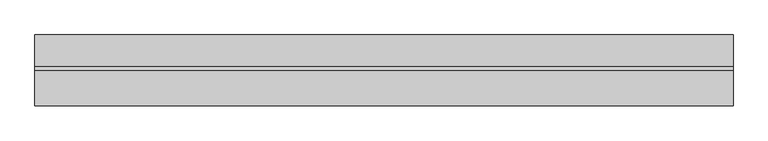
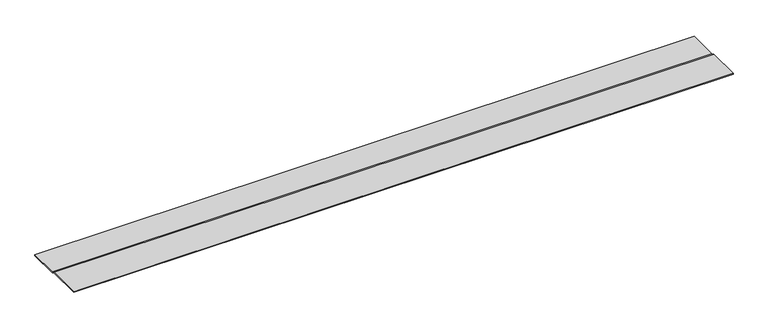
"""IFC4 building model written with IfcOpenShell, lengths in millimetres: proxy geometry, INTERPLY : INTERPLY."""

from ifc_helpers import new_model, si_unit, frame, origin, place, context, project, spatial, polyline, outline, extrude, source, transform, mapped, element, save


def generic_models_e581f4a8(model_context):
    return source(origin(), model_context, "Body", "SweptSolid", [
        extrude(outline(polyline([(-5445.2013056, 40245.4311121), (-5434.635725, 40240.7198889), (-5343.897656, 40240.7198889), (-5343.897656, 40238.4107979), (-5435.1272163, 40238.4107979), (-5445.6927969, 40243.1220211), (-5546.937695, 40243.1220211), (-5546.937695, 40245.4311121), (-5445.2013056, 40245.4311121)])), frame((12382.7678845, 0.0, 0.0), z_axis=(1.0, 0.0, 0.0), x_axis=(0.0, 1.0, 0.0)), (0.0, 0.0, 1.0), 2000.25),
    ])


if __name__ == "__main__":
    model = new_model("IFC4")
    model_context = context("Model", 3, world=origin())
    ifc_project = project(units=[si_unit("LENGTHUNIT", "METRE", prefix="MILLI")], contexts=[model_context])
    site = spatial("IfcSite", under=ifc_project)
    building = spatial("IfcBuilding", under=site)
    placement = place(None, origin())
    generic_models_shape = generic_models_e581f4a8(model_context)
    element("IfcBuildingElementProxy", 1, Name="INTERPLY : INTERPLY", ObjectType="INTERPLY : INTERPLY", at=placement, inside=building, context=model_context, shape_type="MappedRepresentation", body=[
        mapped(generic_models_shape, transform((0.0, 0.0, 0.0), x_axis=(1.0, 0.0, 0.0), y_axis=(0.0, 1.0, 0.0), z_axis=(0.0, 0.0, 1.0))),
    ])
    save(model, "model.ifc")

# Revit data of these elements
# Type "INTERPLY : INTERPLY"
#   NameOverride = "INTERPLY"
# Element 1 (IfcBuildingElementProxy, "INTERPLY : INTERPLY")
#   Materials on its faces: "INTERPLY REQUIRED FOR 15 & 20 YEARS SYSTEMS"
# Materials
#   "INTERPLY REQUIRED FOR 15 & 20 YEARS SYSTEMS": class "Unassigned", colour RGB 115 115 172, transparency 0
